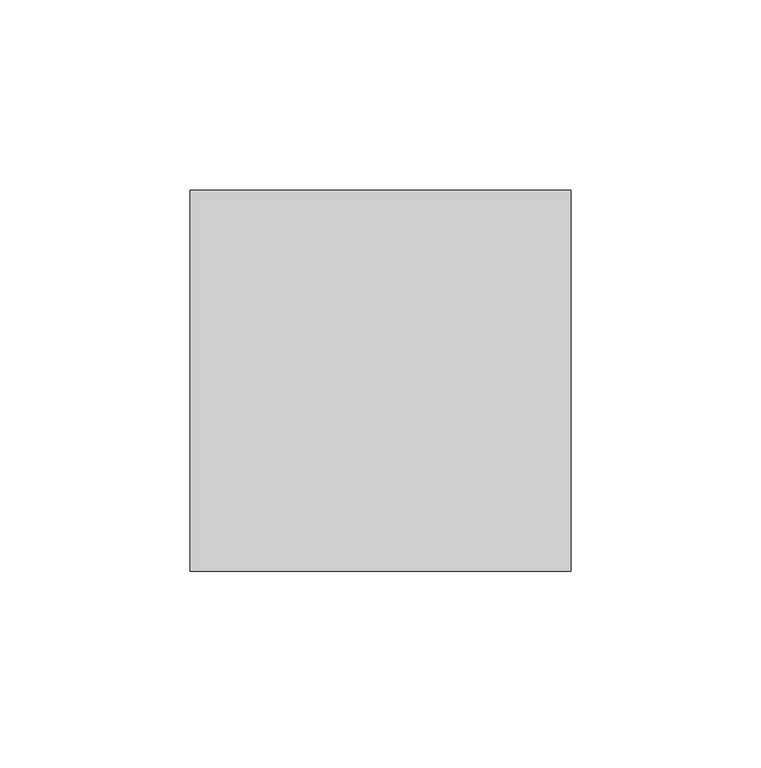
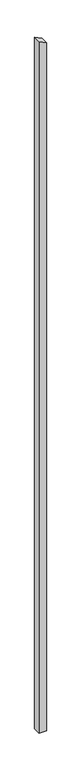
"""IFC4 building model written with IfcOpenShell, lengths in millimetres: column geometry, Holzstütze 158806 : Holzstütze 158806."""

import ifcopenshell
import ifcopenshell.guid

model = None  # the IFC model being written
_history = None  # IfcOwnerHistory: only IFC2X3 demands one
_inside = {}  # id of a spatial element -> (the spatial element, [elements in it])
_under = {}  # id of a project, library or spatial element -> (it, [spatial elements below it])
_declared = {}  # id of a project -> (the project, [libraries it declares])
_typed = {}  # id of a type object -> (the type object, [elements of that type])
_made_of = {}  # id of a material, layer set ... -> (it, [elements and type objects made of it])


def new_model(schema):
    """Start an empty IFC model of exactly this schema.

    Asked for "IFC4X3", IfcOpenShell would pick the latest addendum, in which some entities
    have other attributes; the version numbers below select the first issue.
    IFC2X3 requires an IfcOwnerHistory on every rooted entity: one is made here for all.
    """
    global model, _history
    if schema == "IFC4X3":
        model = ifcopenshell.file(schema_version=(4, 3, 0, 0))
    else:
        model = ifcopenshell.file(schema=schema)
    _inside.clear()
    _under.clear()
    _declared.clear()
    _typed.clear()
    _made_of.clear()
    _history = None
    if model.schema == "IFC2X3":
        org = make("IfcOrganization", Name="unknown")
        user = make(
            "IfcPersonAndOrganization",
            ThePerson=make("IfcPerson", FamilyName="unknown"),
            TheOrganization=org,
        )
        app = make(
            "IfcApplication",
            ApplicationDeveloper=org,
            Version="unknown",
            ApplicationFullName="unknown",
            ApplicationIdentifier="unknown",
        )
        _history = make(
            "IfcOwnerHistory",
            OwningUser=user,
            OwningApplication=app,
            ChangeAction="ADDED",
            CreationDate=0,
        )
    return model


def make(cls, **values):
    """One entity of the class cls with the attributes given. An attribute that is None is left unset."""
    return model.create_entity(
        cls, **{name: value for name, value in values.items() if value is not None}
    )


def rooted(cls, **values):
    """An entity with a GlobalId (a new one), such as an element, a storey or a relation."""
    return make(cls, GlobalId=ifcopenshell.guid.new(), OwnerHistory=_history, **values)


def si_unit(unit_type, name, prefix=None):
    """IfcSIUnit, for example si_unit("LENGTHUNIT", "METRE", prefix="MILLI")."""
    return make("IfcSIUnit", UnitType=unit_type, Prefix=prefix, Name=name)


def assignment(units):
    """IfcUnitAssignment: the units of a project."""
    return None if units is None else make("IfcUnitAssignment", Units=units)


def point(xyz):
    """IfcCartesianPoint."""
    return None if xyz is None else make("IfcCartesianPoint", Coordinates=xyz)


def direction(xyz):
    """IfcDirection."""
    return None if xyz is None else make("IfcDirection", DirectionRatios=xyz)


def frame(location, z_axis=None, x_axis=None):
    """IfcAxis2Placement3D, a coordinate frame: its origin and axes. An axis left out is left unset."""
    return make(
        "IfcAxis2Placement3D",
        Location=point(location),
        Axis=direction(z_axis),
        RefDirection=direction(x_axis),
    )


def origin():
    """The frame at (0, 0, 0) with its axes left unset."""
    return frame((0.0, 0.0, 0.0))


def place(relative_to, where):
    """IfcLocalPlacement: puts the frame where relative to a parent placement (None: the world)."""
    return make(
        "IfcLocalPlacement", PlacementRelTo=relative_to, RelativePlacement=where
    )


def context(
    kind, dimensions, precision=None, world=None, true_north=None, identifier=None
):
    """IfcGeometricRepresentationContext, for example the 3D "Model" context."""
    return make(
        "IfcGeometricRepresentationContext",
        ContextIdentifier=identifier,
        ContextType=kind,
        CoordinateSpaceDimension=dimensions,
        Precision=precision,
        WorldCoordinateSystem=world,
        TrueNorth=true_north,
    )


def project(units=None, contexts=None):
    """IfcProject with its units and contexts."""
    return rooted(
        "IfcProject",
        Name="project",
        RepresentationContexts=contexts,
        UnitsInContext=assignment(units),
    )


def spatial(cls, under=None, at=None, **own):
    """A site, building, storey or space (cls), placed at a placement, below another one or the project."""
    s = rooted(cls, ObjectPlacement=at, **own)
    if under is not None:
        _under.setdefault(under.id(), (under, []))[1].append(s)
    return s


def polyline(points):
    """IfcPolyline through the points."""
    return make("IfcPolyline", Points=[point(p) for p in points])


def outline(outer, holes=None, kind="AREA"):
    """IfcArbitraryClosedProfileDef: a profile drawn as a closed curve; with holes, ...WithVoids."""
    if holes is None:
        return make("IfcArbitraryClosedProfileDef", ProfileType=kind, OuterCurve=outer)
    return make(
        "IfcArbitraryProfileDefWithVoids",
        ProfileType=kind,
        OuterCurve=outer,
        InnerCurves=holes,
    )


def extrude(swept, where, along, depth):
    """IfcExtrudedAreaSolid: the profile swept, set in the frame where, extruded along a direction by depth."""
    return make(
        "IfcExtrudedAreaSolid",
        SweptArea=swept,
        Position=where,
        ExtrudedDirection=direction(along),
        Depth=depth,
    )


def shape(context_of_items, identifier, shape_type, items):
    """IfcShapeRepresentation: the items that make up one representation, for example the "Body"."""
    return make(
        "IfcShapeRepresentation",
        ContextOfItems=context_of_items,
        RepresentationIdentifier=identifier,
        RepresentationType=shape_type,
        Items=items,
    )


def source(mapping_origin, context_of_items, identifier, shape_type, items):
    """IfcRepresentationMap: a shape defined once, which mapped items show again and again."""
    return make(
        "IfcRepresentationMap",
        MappingOrigin=mapping_origin,
        MappedRepresentation=shape(context_of_items, identifier, shape_type, items),
    )


def transform(
    local_origin,
    x_axis=None,
    y_axis=None,
    z_axis=None,
    scale=None,
    scale2=None,
    scale3=None,
    uniform=True,
):
    """IfcCartesianTransformationOperator3D, or its non-uniform kind. x_axis, y_axis, z_axis: its Axis1, 2, 3."""
    if uniform:
        return make(
            "IfcCartesianTransformationOperator3D",
            Axis1=direction(x_axis),
            Axis2=direction(y_axis),
            LocalOrigin=point(local_origin),
            Scale=scale,
            Axis3=direction(z_axis),
        )
    return make(
        "IfcCartesianTransformationOperator3DnonUniform",
        Axis1=direction(x_axis),
        Axis2=direction(y_axis),
        LocalOrigin=point(local_origin),
        Scale=scale,
        Axis3=direction(z_axis),
        Scale2=scale2,
        Scale3=scale3,
    )


def mapped(mapping_source, mapping_target):
    """IfcMappedItem: shows the shape of a source again, moved by a transform."""
    return make(
        "IfcMappedItem", MappingSource=mapping_source, MappingTarget=mapping_target
    )


def made_of(thing, what):
    """Note that an element or type object is made of a material, layer set ...; save() writes the relation."""
    if what is not None:
        _made_of.setdefault(what.id(), (what, []))[1].append(thing)
    return thing


def element(
    cls,
    number,
    at=None,
    inside=None,
    cuts=None,
    type_object=None,
    material=None,
    context=None,
    identifier="Body",
    shape_type=None,
    held_by="IfcProductDefinitionShape",
    body=None,
    shapes=None,
    **own,
):
    """One element of the class cls, such as IfcWall. Its Tag is "e" and its number.

    at: its placement. inside: the storey or other place that contains it. cuts: it is an
    opening in that element (IfcRelVoidsElement). A single representation is given by context,
    identifier, shape_type and body (its items); several are given by shapes. held_by: the class
    of the entity that holds the representations. save() writes the other relations.
    """
    e = rooted(cls, Tag="e%d" % number, ObjectPlacement=at, **own)
    if body is not None:
        shapes = [shape(context, identifier, shape_type, body)]
    if shapes is not None:
        e.Representation = make(held_by, Representations=shapes)
    if inside is not None:
        _inside.setdefault(inside.id(), (inside, []))[1].append(e)
    if cuts is not None:
        rooted(
            "IfcRelVoidsElement", RelatingBuildingElement=cuts, RelatedOpeningElement=e
        )
    if type_object is not None:
        _typed.setdefault(type_object.id(), (type_object, []))[1].append(e)
    return made_of(e, material)


def aggregate(whole, parts):
    """IfcRelAggregates: a whole, such as a stair, and the parts it consists of."""
    return rooted("IfcRelAggregates", RelatingObject=whole, RelatedObjects=parts)


def save(model, path):
    """Write the relations noted so far, then the file.

    IfcRelAggregates (storeys below a building ...), IfcRelContainedInSpatialStructure (elements
    in a storey), IfcRelDefinesByType, IfcRelAssociatesMaterial and IfcRelDeclares: one each for
    every whole, place, type object, material and project.
    """
    for whole, parts in _under.values():
        aggregate(whole, parts)
    for where, things in _inside.values():
        rooted(
            "IfcRelContainedInSpatialStructure",
            RelatedElements=things,
            RelatingStructure=where,
        )
    for kind, things in _typed.values():
        rooted("IfcRelDefinesByType", RelatedObjects=things, RelatingType=kind)
    for what, things in _made_of.values():
        rooted("IfcRelAssociatesMaterial", RelatedObjects=things, RelatingMaterial=what)
    for by, libraries in _declared.values():
        rooted("IfcRelDeclares", RelatingContext=by, RelatedDefinitions=libraries)
    model.write(path)


def column_4e503af9(model_context):
    return source(origin(), model_context, "Body", "SweptSolid", [
        extrude(outline(polyline([(-500.0, 168257.7593015), (-500.0, 168357.7593015), (9372.2929958, 168357.7593015), (9423.2455407, 168257.7593015), (-500.0, 168257.7593015)])), frame((0.0, 47884.7962965, 0.0), z_axis=(0.0, 1.0, 0.0), x_axis=(0.0, 0.0, 1.0)), (0.0, 0.0, 1.0), 100.0),
    ])


if __name__ == "__main__":
    model = new_model("IFC4")
    model_context = context("Model", 3, world=origin())
    ifc_project = project(units=[si_unit("LENGTHUNIT", "METRE", prefix="MILLI")], contexts=[model_context])
    site = spatial("IfcSite", under=ifc_project)
    building = spatial("IfcBuilding", under=site)
    placement = place(None, origin())
    column_shape = column_4e503af9(model_context)
    element("IfcColumn", 1, ObjectType="Holzstütze 158806 : Holzstütze 158806", at=placement, inside=building, context=model_context, shape_type="MappedRepresentation", body=[
        mapped(column_shape, transform((0.0, 0.0, 0.0), x_axis=(1.0, 0.0, 0.0), y_axis=(0.0, 1.0, 0.0), z_axis=(0.0, 0.0, 1.0))),
    ])
    save(model, "model.ifc")

# Revit data of these elements
# Type "Holzstütze 158806 : Holzstütze 158806"
#   Abrechnungsart = "m"
#   Allright_Bauteil_ID = "0152St 0000143380"
#   Bezeichnung = "Holzstütze"
#   Codetext = "ST-HOLZ\\"
#   Gewerk = "Zimmer- und Holzbauarbeiten"
#   Material = "Holz"
#   Objektname = "Stütze"
#   NameOverride = "Holzstütze"
#   Reference = "Holzstütze"
#   Status = "NEW"
#   ThermalTransmittance = 0.0000 BTU/(h·ft²·°F)
#   Roll = 0.00°
#   Slope = 0.00°
#   2D Interaktion = yes
#   IsExternal = yes
#   LoadBearing = yes
# Element 1 (IfcColumn, "Holzstütze 158806 : Holzstütze 158806")
#   Materials on its faces: "holzschalung"
# Materials
#   "holzschalung": class "Unassigned", colour RGB 128 128 128, transparency 0
